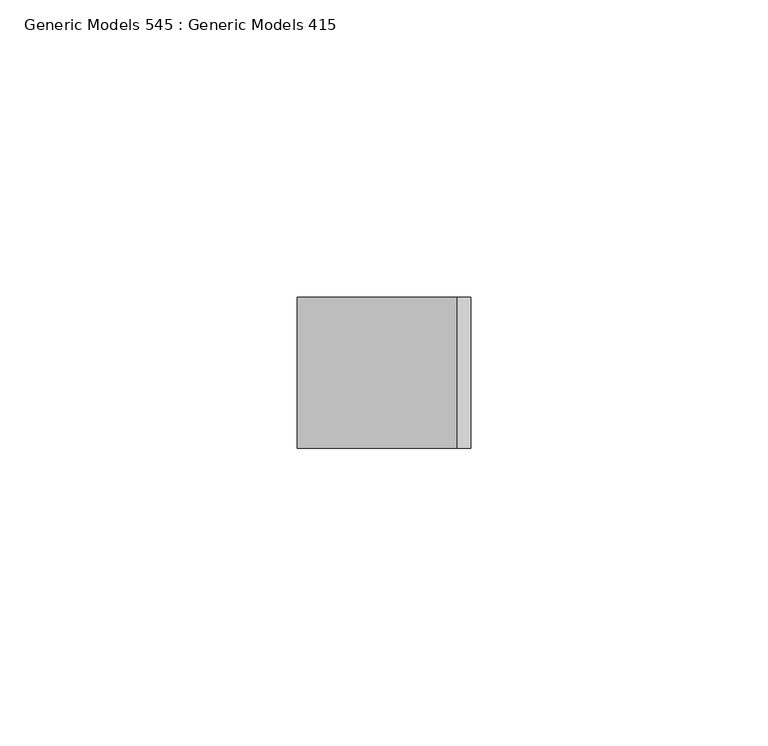
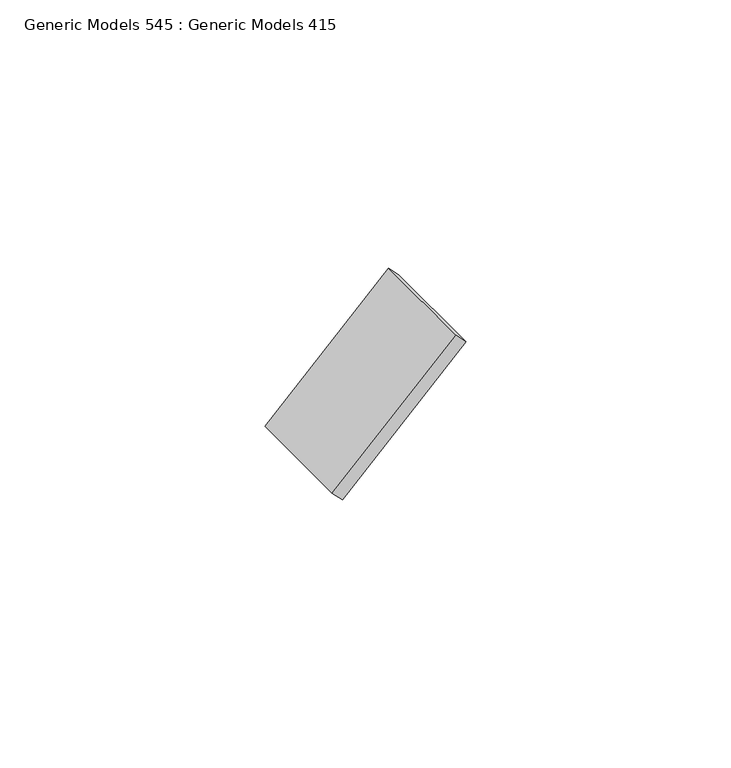
"""IFC4 building model written with IfcOpenShell, lengths in millimetres: proxy geometry, Generic Models 545 : Generic Models 415."""

from ifc_helpers import new_model, si_unit, frame, origin, place, context, project, spatial, polyline, outline, extrude, source, transform, mapped, element, save


def generic_models_545_generic_models_415_37b518b4(model_context):
    return source(origin(), model_context, "Body", "SweptSolid", [
        extrude(outline(polyline([(0.0, -3.175), (0.0, 0.0), (25.4, 0.0), (25.4, -3.175), (0.0, -3.175)])), frame((7848.0411784, 4501.3863946, 124876.8849742), z_axis=(0.7071067811867181, 0.0, 0.707106781186377), x_axis=(0.0, -1.0, 0.0)), (0.0, 0.0, 1.0), 38.1),
    ])


if __name__ == "__main__":
    model = new_model("IFC4")
    model_context = context("Model", 3, world=origin())
    ifc_project = project(units=[si_unit("LENGTHUNIT", "METRE", prefix="MILLI")], contexts=[model_context])
    site = spatial("IfcSite", under=ifc_project)
    building = spatial("IfcBuilding", under=site)
    placement = place(None, origin())
    generic_models_545_generic_models_415_shape = generic_models_545_generic_models_415_37b518b4(model_context)
    element("IfcBuildingElementProxy", 1, Name="Generic Models 545 : Generic Models 415", ObjectType="Generic Models 545 : Generic Models 415", at=placement, inside=building, context=model_context, shape_type="MappedRepresentation", body=[
        mapped(generic_models_545_generic_models_415_shape, transform((0.0, 0.0, 0.0), x_axis=(1.0, 0.0, 0.0), y_axis=(0.0, 1.0, 0.0), z_axis=(0.0, 0.0, 1.0))),
    ])
    save(model, "model.ifc")

# Revit data of these elements
# Element 1 (IfcBuildingElementProxy, "Generic Models 545 : Generic Models 415")
#   Materials on its faces: "_WELDED STEEL TABS FOR LOUVER ATTACHMENT"
# Materials
#   "_WELDED STEEL TABS FOR LOUVER ATTACHMENT": class "Metal", colour RGB 199 199 199, transparency 0, Description = "Structural steel 50ksi", Cost = 0
